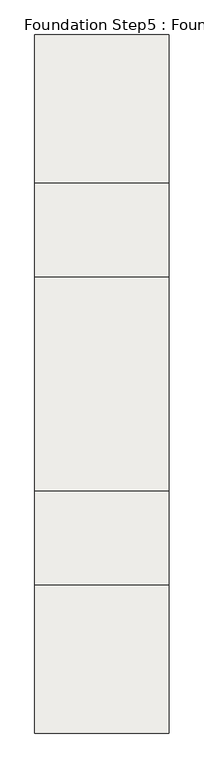
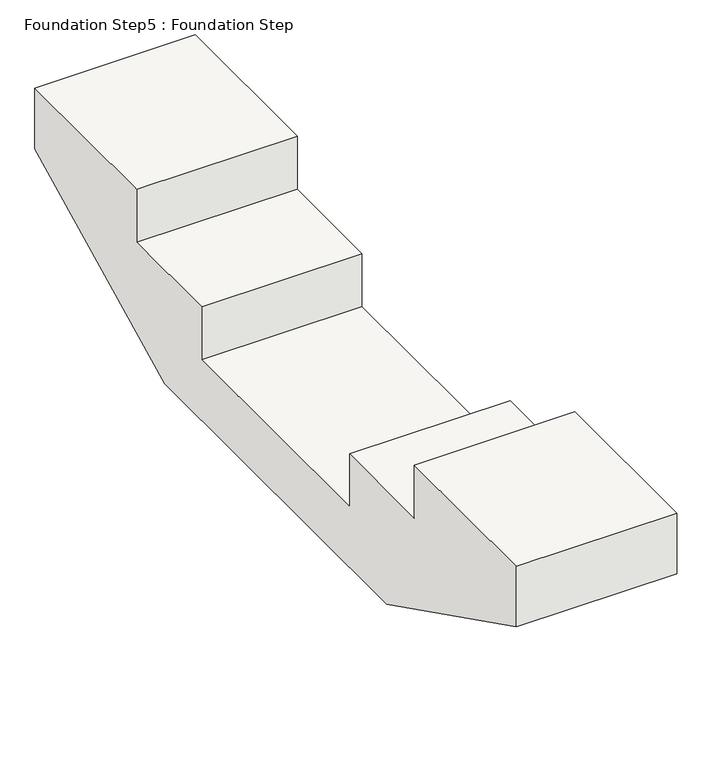
"""IFC4 building model written with IfcOpenShell, lengths in millimetres: slab geometry, Foundation Step5 : Foundation Step."""

from ifc_helpers import new_model, si_unit, frame, origin, place, context, project, spatial, polyline, outline, extrude, source, transform, mapped, element, save


def foundation_step5_foundation_step_64dcdb90(model_context):
    return source(origin(), model_context, "Body", "SweptSolid", [
        extrude(outline(polyline([(-538.4231529, -1092.2), (299.7768471, -1092.2), (299.7768471, -1358.9), (833.1768471, -1358.9), (833.1768471, -1625.6), (2052.3768471, -1625.6), (2052.3768471, -1358.9), (2585.7768471, -1358.9), (2585.7768471, -1092.2), (3423.9768471, -1092.2), (3423.9768471, -1397.0), (2357.1768471, -1930.4), (528.3768471, -1930.4), (-538.4231529, -1397.0), (-538.4231529, -1092.2)])), frame((-49531.6350821, 0.0, 0.0), z_axis=(1.0, 0.0, 0.0), x_axis=(0.0, 1.0, 0.0)), (0.0, 0.0, 1.0), 762.0),
    ])


if __name__ == "__main__":
    model = new_model("IFC4")
    model_context = context("Model", 3, world=origin())
    ifc_project = project(units=[si_unit("LENGTHUNIT", "METRE", prefix="MILLI")], contexts=[model_context])
    site = spatial("IfcSite", under=ifc_project)
    building = spatial("IfcBuilding", under=site)
    placement = place(None, origin())
    foundation_step5_foundation_step_shape = foundation_step5_foundation_step_64dcdb90(model_context)
    element("IfcSlab", 1, ObjectType="Foundation Step5 : Foundation Step", at=placement, inside=building, context=model_context, shape_type="MappedRepresentation", body=[
        mapped(foundation_step5_foundation_step_shape, transform((0.0, 0.0, 0.0), x_axis=(1.0, 0.0, 0.0), y_axis=(0.0, 1.0, 0.0), z_axis=(0.0, 0.0, 1.0))),
    ])
    save(model, "model.ifc")

# Revit data of these elements
# Type "Foundation Step5 : Foundation Step"
#   Structural Material = Concrete, Cast-in-Place gray
# Materials
#   "Concrete, Cast-in-Place gray": class "Concrete", colour RGB 192 192 192, transparency 0, Description = "Cast-in-place concrete", Cost = 0
